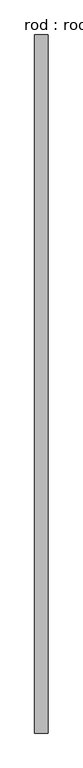
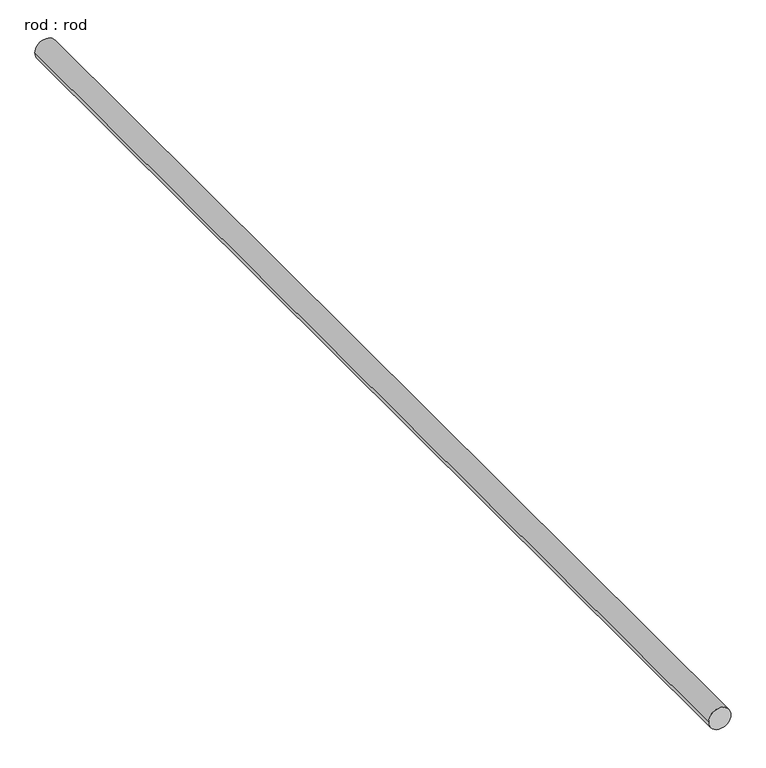
"""IFC4 building model written with IfcOpenShell, lengths in millimetres: proxy geometry, rod : rod."""

from ifc_helpers import new_model, si_unit, point, frame, frame_2d, origin, place, context, project, spatial, circle_curve, trimmed, segment, composite_curve, outline, extrude, source, transform, mapped, element, save


def rod_rod_a2558ae4(model_context):
    return source(origin(), model_context, "Body", "SweptSolid", [
        extrude(outline(composite_curve([segment(trimmed(circle_curve(frame_2d((0.0108462, 0.0)), 200.0), [point((0.0108462, 200.0))], [point((0.0108462, -200.0))], False, "CARTESIAN"), True, "CONTINUOUS"), segment(trimmed(circle_curve(frame_2d((0.0108462, 0.0)), 200.0), [point((0.0108462, -200.0))], [point((0.0108462, 200.0))], False, "CARTESIAN"), True, "CONTINUOUS")], self_intersect=False)), frame((0.0, -6385.6804361, 0.0), z_axis=(0.0, 1.0, 0.0), x_axis=(0.0, 0.0, 1.0)), (0.0, 0.0, 1.0), 20956.8181029),
    ])


if __name__ == "__main__":
    model = new_model("IFC4")
    model_context = context("Model", 3, world=origin())
    ifc_project = project(units=[si_unit("LENGTHUNIT", "METRE", prefix="MILLI")], contexts=[model_context])
    site = spatial("IfcSite", under=ifc_project)
    building = spatial("IfcBuilding", under=site)
    placement = place(None, origin())
    rod_rod_shape = rod_rod_a2558ae4(model_context)
    element("IfcBuildingElementProxy", 1, Name="rod : rod", ObjectType="rod : rod", at=placement, inside=building, context=model_context, shape_type="MappedRepresentation", body=[
        mapped(rod_rod_shape, transform((0.0, 0.0, 0.0), x_axis=(1.0, 0.0, 0.0), y_axis=(0.0, 1.0, 0.0), z_axis=(0.0, 0.0, 1.0))),
    ])
    save(model, "model.ifc")

# Revit data of these elements
# Type "rod : rod"
#   Default Elevation = 0
